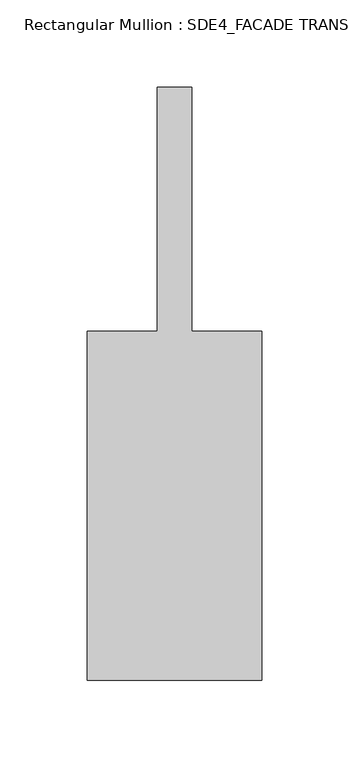
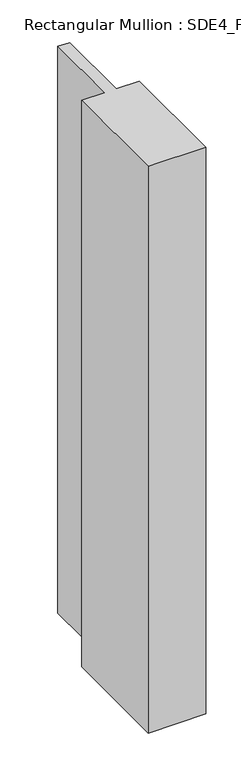
"""IFC4 building model written with IfcOpenShell, lengths in millimetres: member geometry, Rectangular Mullion : SDE4_FACADE TRANSOM TYPE 1."""

import ifcopenshell
import ifcopenshell.guid

model = None  # the IFC model being written
_history = None  # IfcOwnerHistory: only IFC2X3 demands one
_inside = {}  # id of a spatial element -> (the spatial element, [elements in it])
_under = {}  # id of a project, library or spatial element -> (it, [spatial elements below it])
_declared = {}  # id of a project -> (the project, [libraries it declares])
_typed = {}  # id of a type object -> (the type object, [elements of that type])
_made_of = {}  # id of a material, layer set ... -> (it, [elements and type objects made of it])


def new_model(schema):
    """Start an empty IFC model of exactly this schema.

    Asked for "IFC4X3", IfcOpenShell would pick the latest addendum, in which some entities
    have other attributes; the version numbers below select the first issue.
    IFC2X3 requires an IfcOwnerHistory on every rooted entity: one is made here for all.
    """
    global model, _history
    if schema == "IFC4X3":
        model = ifcopenshell.file(schema_version=(4, 3, 0, 0))
    else:
        model = ifcopenshell.file(schema=schema)
    _inside.clear()
    _under.clear()
    _declared.clear()
    _typed.clear()
    _made_of.clear()
    _history = None
    if model.schema == "IFC2X3":
        org = make("IfcOrganization", Name="unknown")
        user = make(
            "IfcPersonAndOrganization",
            ThePerson=make("IfcPerson", FamilyName="unknown"),
            TheOrganization=org,
        )
        app = make(
            "IfcApplication",
            ApplicationDeveloper=org,
            Version="unknown",
            ApplicationFullName="unknown",
            ApplicationIdentifier="unknown",
        )
        _history = make(
            "IfcOwnerHistory",
            OwningUser=user,
            OwningApplication=app,
            ChangeAction="ADDED",
            CreationDate=0,
        )
    return model


def make(cls, **values):
    """One entity of the class cls with the attributes given. An attribute that is None is left unset."""
    return model.create_entity(
        cls, **{name: value for name, value in values.items() if value is not None}
    )


def rooted(cls, **values):
    """An entity with a GlobalId (a new one), such as an element, a storey or a relation."""
    return make(cls, GlobalId=ifcopenshell.guid.new(), OwnerHistory=_history, **values)


def si_unit(unit_type, name, prefix=None):
    """IfcSIUnit, for example si_unit("LENGTHUNIT", "METRE", prefix="MILLI")."""
    return make("IfcSIUnit", UnitType=unit_type, Prefix=prefix, Name=name)


def assignment(units):
    """IfcUnitAssignment: the units of a project."""
    return None if units is None else make("IfcUnitAssignment", Units=units)


def point(xyz):
    """IfcCartesianPoint."""
    return None if xyz is None else make("IfcCartesianPoint", Coordinates=xyz)


def direction(xyz):
    """IfcDirection."""
    return None if xyz is None else make("IfcDirection", DirectionRatios=xyz)


def frame(location, z_axis=None, x_axis=None):
    """IfcAxis2Placement3D, a coordinate frame: its origin and axes. An axis left out is left unset."""
    return make(
        "IfcAxis2Placement3D",
        Location=point(location),
        Axis=direction(z_axis),
        RefDirection=direction(x_axis),
    )


def origin():
    """The frame at (0, 0, 0) with its axes left unset."""
    return frame((0.0, 0.0, 0.0))


def place(relative_to, where):
    """IfcLocalPlacement: puts the frame where relative to a parent placement (None: the world)."""
    return make(
        "IfcLocalPlacement", PlacementRelTo=relative_to, RelativePlacement=where
    )


def context(
    kind, dimensions, precision=None, world=None, true_north=None, identifier=None
):
    """IfcGeometricRepresentationContext, for example the 3D "Model" context."""
    return make(
        "IfcGeometricRepresentationContext",
        ContextIdentifier=identifier,
        ContextType=kind,
        CoordinateSpaceDimension=dimensions,
        Precision=precision,
        WorldCoordinateSystem=world,
        TrueNorth=true_north,
    )


def project(units=None, contexts=None):
    """IfcProject with its units and contexts."""
    return rooted(
        "IfcProject",
        Name="project",
        RepresentationContexts=contexts,
        UnitsInContext=assignment(units),
    )


def spatial(cls, under=None, at=None, **own):
    """A site, building, storey or space (cls), placed at a placement, below another one or the project."""
    s = rooted(cls, ObjectPlacement=at, **own)
    if under is not None:
        _under.setdefault(under.id(), (under, []))[1].append(s)
    return s


def polyline(points):
    """IfcPolyline through the points."""
    return make("IfcPolyline", Points=[point(p) for p in points])


def outline(outer, holes=None, kind="AREA"):
    """IfcArbitraryClosedProfileDef: a profile drawn as a closed curve; with holes, ...WithVoids."""
    if holes is None:
        return make("IfcArbitraryClosedProfileDef", ProfileType=kind, OuterCurve=outer)
    return make(
        "IfcArbitraryProfileDefWithVoids",
        ProfileType=kind,
        OuterCurve=outer,
        InnerCurves=holes,
    )


def extrude(swept, where, along, depth):
    """IfcExtrudedAreaSolid: the profile swept, set in the frame where, extruded along a direction by depth."""
    return make(
        "IfcExtrudedAreaSolid",
        SweptArea=swept,
        Position=where,
        ExtrudedDirection=direction(along),
        Depth=depth,
    )


def shape(context_of_items, identifier, shape_type, items):
    """IfcShapeRepresentation: the items that make up one representation, for example the "Body"."""
    return make(
        "IfcShapeRepresentation",
        ContextOfItems=context_of_items,
        RepresentationIdentifier=identifier,
        RepresentationType=shape_type,
        Items=items,
    )


def source(mapping_origin, context_of_items, identifier, shape_type, items):
    """IfcRepresentationMap: a shape defined once, which mapped items show again and again."""
    return make(
        "IfcRepresentationMap",
        MappingOrigin=mapping_origin,
        MappedRepresentation=shape(context_of_items, identifier, shape_type, items),
    )


def transform(
    local_origin,
    x_axis=None,
    y_axis=None,
    z_axis=None,
    scale=None,
    scale2=None,
    scale3=None,
    uniform=True,
):
    """IfcCartesianTransformationOperator3D, or its non-uniform kind. x_axis, y_axis, z_axis: its Axis1, 2, 3."""
    if uniform:
        return make(
            "IfcCartesianTransformationOperator3D",
            Axis1=direction(x_axis),
            Axis2=direction(y_axis),
            LocalOrigin=point(local_origin),
            Scale=scale,
            Axis3=direction(z_axis),
        )
    return make(
        "IfcCartesianTransformationOperator3DnonUniform",
        Axis1=direction(x_axis),
        Axis2=direction(y_axis),
        LocalOrigin=point(local_origin),
        Scale=scale,
        Axis3=direction(z_axis),
        Scale2=scale2,
        Scale3=scale3,
    )


def mapped(mapping_source, mapping_target):
    """IfcMappedItem: shows the shape of a source again, moved by a transform."""
    return make(
        "IfcMappedItem", MappingSource=mapping_source, MappingTarget=mapping_target
    )


def made_of(thing, what):
    """Note that an element or type object is made of a material, layer set ...; save() writes the relation."""
    if what is not None:
        _made_of.setdefault(what.id(), (what, []))[1].append(thing)
    return thing


def element(
    cls,
    number,
    at=None,
    inside=None,
    cuts=None,
    type_object=None,
    material=None,
    context=None,
    identifier="Body",
    shape_type=None,
    held_by="IfcProductDefinitionShape",
    body=None,
    shapes=None,
    **own,
):
    """One element of the class cls, such as IfcWall. Its Tag is "e" and its number.

    at: its placement. inside: the storey or other place that contains it. cuts: it is an
    opening in that element (IfcRelVoidsElement). A single representation is given by context,
    identifier, shape_type and body (its items); several are given by shapes. held_by: the class
    of the entity that holds the representations. save() writes the other relations.
    """
    e = rooted(cls, Tag="e%d" % number, ObjectPlacement=at, **own)
    if body is not None:
        shapes = [shape(context, identifier, shape_type, body)]
    if shapes is not None:
        e.Representation = make(held_by, Representations=shapes)
    if inside is not None:
        _inside.setdefault(inside.id(), (inside, []))[1].append(e)
    if cuts is not None:
        rooted(
            "IfcRelVoidsElement", RelatingBuildingElement=cuts, RelatedOpeningElement=e
        )
    if type_object is not None:
        _typed.setdefault(type_object.id(), (type_object, []))[1].append(e)
    return made_of(e, material)


def aggregate(whole, parts):
    """IfcRelAggregates: a whole, such as a stair, and the parts it consists of."""
    return rooted("IfcRelAggregates", RelatingObject=whole, RelatedObjects=parts)


def save(model, path):
    """Write the relations noted so far, then the file.

    IfcRelAggregates (storeys below a building ...), IfcRelContainedInSpatialStructure (elements
    in a storey), IfcRelDefinesByType, IfcRelAssociatesMaterial and IfcRelDeclares: one each for
    every whole, place, type object, material and project.
    """
    for whole, parts in _under.values():
        aggregate(whole, parts)
    for where, things in _inside.values():
        rooted(
            "IfcRelContainedInSpatialStructure",
            RelatedElements=things,
            RelatingStructure=where,
        )
    for kind, things in _typed.values():
        rooted("IfcRelDefinesByType", RelatedObjects=things, RelatingType=kind)
    for what, things in _made_of.values():
        rooted("IfcRelAssociatesMaterial", RelatedObjects=things, RelatingMaterial=what)
    for by, libraries in _declared.values():
        rooted("IfcRelDeclares", RelatingContext=by, RelatedDefinitions=libraries)
    model.write(path)


def rectangular_mullion_sde4_facade_transom_type_1_a8214493(model_context):
    return source(origin(), model_context, "Body", "SweptSolid", [
        extrude(outline(polyline([(50.0, -132.5), (-50.0, -132.5), (-50.0, 67.5), (-10.0, 67.5), (-10.0, 207.5), (10.0, 207.5), (10.0, 67.5), (50.0, 67.5), (50.0, -132.5)])), frame((0.0, 0.0, -1039.0), z_axis=(0.0, 0.0, 1.0), x_axis=(1.0, 0.0, 0.0)), (0.0, 0.0, 1.0), 1039.0),
    ])


if __name__ == "__main__":
    model = new_model("IFC4")
    model_context = context("Model", 3, world=origin())
    ifc_project = project(units=[si_unit("LENGTHUNIT", "METRE", prefix="MILLI")], contexts=[model_context])
    site = spatial("IfcSite", under=ifc_project)
    building = spatial("IfcBuilding", under=site)
    placement = place(None, origin())
    rectangular_mullion_sde4_facade_transom_type_1_shape = rectangular_mullion_sde4_facade_transom_type_1_a8214493(model_context)
    element("IfcMember", 1, ObjectType="Rectangular Mullion : SDE4_FACADE TRANSOM TYPE 1", at=placement, inside=building, context=model_context, shape_type="MappedRepresentation", body=[
        mapped(rectangular_mullion_sde4_facade_transom_type_1_shape, transform((0.0, 0.0, 0.0), x_axis=(1.0, 0.0, 0.0), y_axis=(0.0, 1.0, 0.0), z_axis=(0.0, 0.0, 1.0))),
    ])
    save(model, "model.ifc")

# Revit data of these elements
# Type "Rectangular Mullion : SDE4_FACADE TRANSOM TYPE 1"
#   built-in parameter 1007322 = 1.11549 (stored number, unit not read)
#   built-in parameter 1007321 = 0.164042 (stored number, unit not read)
#   built-in parameter 1007320 = 0.164042 (stored number, unit not read)
